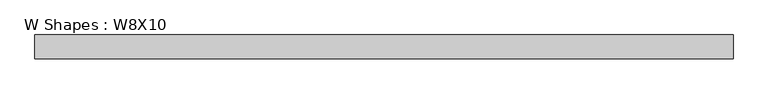
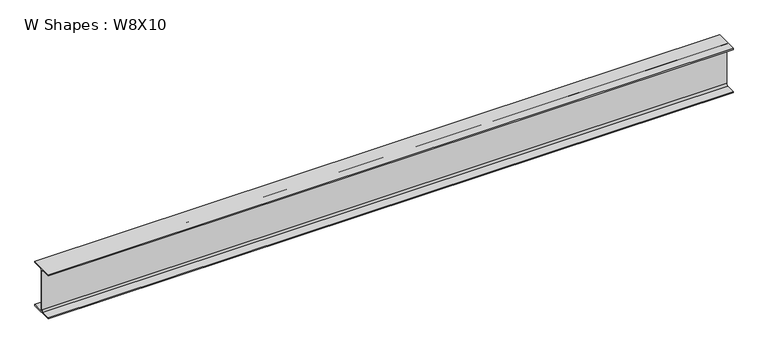
"""IFC4 building model written with IfcOpenShell, lengths in millimetres: beam geometry, W Shapes : W8X10."""

from ifc_helpers import new_model, si_unit, point, frame, frame_2d, origin, place, context, project, spatial, polyline, circle_curve, trimmed, segment, composite_curve, outline, extrude, source, transform, mapped, element, save


def w_shapes_w8x10_60410601(model_context):
    return source(origin(), model_context, "Body", "SweptSolid", [
        extrude(outline(composite_curve([segment(polyline([(50.038, -94.869), (50.038, -100.203), (-50.038, -100.203), (-50.038, -94.869), (-9.779, -94.869)]), True, "CONTINUOUS"), segment(trimmed(circle_curve(frame_2d((-9.779, -87.249)), 7.62), [point((-9.779, -94.869))], [point((-2.159, -87.249))], True, "CARTESIAN"), True, "CONTINUOUS"), segment(polyline([(-2.159, -87.249), (-2.159, 87.249)]), True, "CONTINUOUS"), segment(trimmed(circle_curve(frame_2d((-9.779, 87.249)), 7.62), [point((-2.159, 87.249))], [point((-9.779, 94.869))], True, "CARTESIAN"), True, "CONTINUOUS"), segment(polyline([(-9.779, 94.869), (-50.038, 94.869), (-50.038, 100.203), (50.038, 100.203), (50.038, 94.869), (9.779, 94.869)]), True, "CONTINUOUS"), segment(trimmed(circle_curve(frame_2d((9.779, 87.249)), 7.62), [point((9.779, 94.869))], [point((2.159, 87.249))], True, "CARTESIAN"), True, "CONTINUOUS"), segment(polyline([(2.159, 87.249), (2.159, -87.249)]), True, "CONTINUOUS"), segment(trimmed(circle_curve(frame_2d((9.779, -87.249)), 7.62), [point((2.159, -87.249))], [point((9.779, -94.869))], True, "CARTESIAN"), True, "CONTINUOUS"), segment(polyline([(9.779, -94.869), (50.038, -94.869)]), True, "CONTINUOUS")], self_intersect=False)), frame((-1461.262, 0.0, 0.0), z_axis=(1.0, 0.0, 0.0), x_axis=(0.0, 1.0, 0.0)), (0.0, 0.0, 1.0), 2922.524),
    ])


if __name__ == "__main__":
    model = new_model("IFC4")
    model_context = context("Model", 3, world=origin())
    ifc_project = project(units=[si_unit("LENGTHUNIT", "METRE", prefix="MILLI")], contexts=[model_context])
    site = spatial("IfcSite", under=ifc_project)
    building = spatial("IfcBuilding", under=site)
    placement = place(None, origin())
    w_shapes_w8x10_shape = w_shapes_w8x10_60410601(model_context)
    element("IfcBeam", 1, ObjectType="W Shapes : W8X10", at=placement, inside=building, context=model_context, shape_type="MappedRepresentation", body=[
        mapped(w_shapes_w8x10_shape, transform((0.0, 0.0, 0.0), x_axis=(1.0, 0.0, 0.0), y_axis=(0.0, 1.0, 0.0), z_axis=(0.0, 0.0, 1.0))),
    ])
    save(model, "model.ifc")

# Revit data of these elements
# Type "W Shapes : W8X10"
#   Section Name Key = "W8x10"
#   Assembly Code = "B10"
#   Width = 100.076 mm
#   Web Thickness = 4.318 mm
#   Web Fillet = 7.62 mm
#   Warping Constant = 8297.76 cm⁶
#   Torsional Moment of Inertia = 1.77315 cm⁴
#   Section Area = 2.96 in²
#   Plastic Modulus weak axis = 0.000960648 (stored number, unit not read)
#   Plastic Modulus strong axis = 0.0051331 (stored number, unit not read)
#   Perimeter = 9.35736 m²/m
#   Nominal Weight = 145.939 N/m
#   Moment of Inertia weak axis = 86.9924 cm⁴
#   Moment of Inertia strong axis = 1281.99 cm⁴
#   Height = 200.406 mm
#   Flange Thickness = 5.334 mm
#   Elastic Modulus weak axis = 0.000613426 (stored number, unit not read)
#   Elastic Modulus strong axis = 0.00451968 (stored number, unit not read)
#   Centroid Vertical = 100.203 mm
#   Centroid Horizontal = 50.038 mm
#   Length [instance default] = 5' - 0"
#   Structural Material [instance default] = Steel ASTM A992
#   Principal Axes Angle = 0
# Element 1 (IfcBeam, "W Shapes : W8X10")
#   Materials on its faces: "Steel ASTM A992"
# Materials
#   "Steel ASTM A992": class "Metal", colour RGB 199 199 199, transparency 0, Description = "Structural steel 50ksi", Cost = 0
